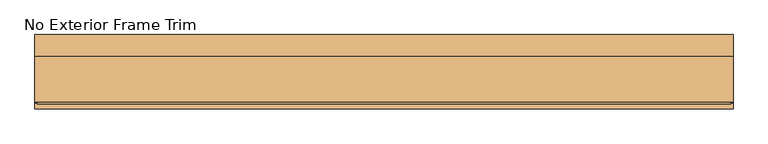
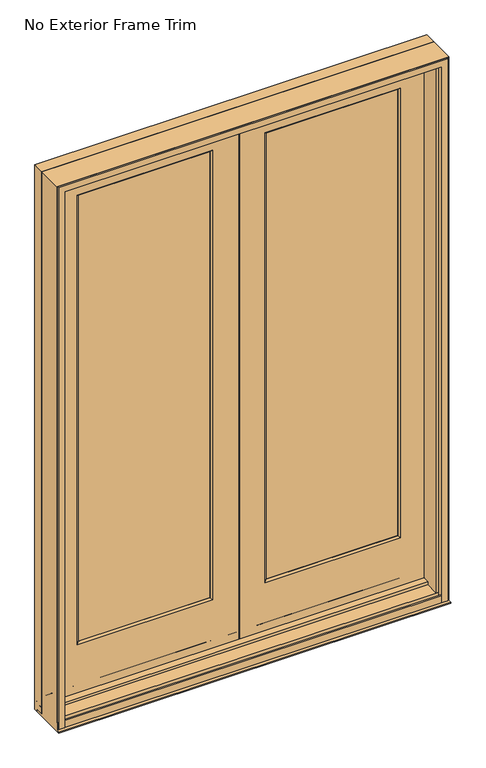
"""IFC4 building model written with IfcOpenShell, lengths in millimetres: door geometry, Door-In_Swing-Milgard-Essence-2_Panel : No Exterior Frame Trim."""

from ifc_helpers import new_model, si_unit, frame, origin, place, context, project, spatial, polyline, outline, extrude, faceted_brep, source, transform, mapped, element, save


def no_exterior_frame_trim_7f6cfa7b(model_context):
    return source(origin(), model_context, "Body", "SolidModel", [
        extrude(outline(polyline([(591.4684989, 28.575), (54.2422052, 28.575), (54.2422052, 53.975), (591.4684989, 53.975), (591.4684989, 28.575)])), frame((0.0, 0.0, 245.0465023), z_axis=(0.0, 0.0, 1.0), x_axis=(1.0, 0.0, 0.0)), (0.0, 0.0, 1.0), 1856.965426),
        faceted_brep([(-22.501829, 56.3244996, 39.0524923), (-39.8139839, 56.3244996, 39.0524923), (-39.8139839, 64.6430002, 39.0524923), (685.524688, 64.6430002, 39.0524923), (685.524688, 56.3244996, 39.0524923), (668.2125331, 56.3244996, 39.0524923), (665.7443122, 53.2765006, 39.0524923), (597.9581931, 53.2765006, 39.0524923), (597.9581931, 55.0418002, 39.0524923), (583.7647037, 55.0418002, 39.0524923), (582.2411552, 53.975, 39.0524923), (578.7581009, 53.975, 39.0524923), (578.7581009, 55.857139, 39.0524923), (579.0279319, 56.3244996, 39.0524923), (66.6827722, 56.3244996, 39.0524923), (66.9526032, 55.857139, 39.0524923), (66.9526032, 53.975, 39.0524923), (63.4695489, 53.975, 39.0524923), (61.9460004, 55.0418002, 39.0524923), (47.7525111, 55.0418002, 39.0524923), (47.7525111, 53.2765006, 39.0524923), (-20.0336081, 53.2765006, 39.0524923), (-22.501829, 56.3244996, 2178.7559624), (-22.501829, 56.3244996, 257.4235308), (-22.1233678, 55.857139, 257.6933617), (-20.5992417, 53.975, 257.6933617), (-20.5992417, 53.975, 254.2103075), (-21.4631194, 55.0418002, 252.686759), (-21.4631194, 55.0418002, 238.4932696), (-20.0336081, 53.2765006, 238.4932696), (-20.0336081, 53.2765006, 2176.2877415), (-20.0336081, 53.2765006, 58.8285873), (-22.501829, 56.3244996, 56.3603664), (47.7525111, 53.2765006, 58.8285873), (597.9581931, 53.2765006, 58.8285873), (665.7443122, 53.2765006, 58.8285873), (685.524688, 53.2765006, 58.8285873), (685.524688, 53.2765006, 238.4932696), (665.7443122, 53.2765006, 238.4932696), (665.7443122, 53.2765006, 2176.2877415), (-39.8139839, 53.2765006, 238.4932696), (-39.8139839, 53.2765006, 58.8285873), (47.7525111, 53.2765006, 2108.5016224), (597.9581931, 53.2765006, 2108.5016224), (597.9581931, 53.2765006, 238.4932696), (47.7525111, 53.2765006, 238.4932696), (47.7525111, 55.0418002, 238.4932696), (47.7525111, 55.0418002, 252.686759), (47.7525111, 53.975, 254.2103075), (47.7525111, 53.975, 257.6933617), (47.7525111, 55.0418002, 257.6933617), (47.7525111, 55.0418002, 2108.5016224), (47.7525111, 55.0418002, 57.3990759), (597.9581931, 55.0418002, 57.3990759), (583.7647037, 55.0418002, 57.3990759), (61.9460004, 55.0418002, 238.4932696), (61.9460004, 55.0418002, 252.686759), (61.9460004, 55.0418002, 257.6933617), (61.9460004, 55.0418002, 2094.3081331), (583.7647037, 55.0418002, 2094.3081331), (583.7647037, 55.0418002, 257.6933617), (597.9581931, 55.0418002, 257.6933617), (597.9581931, 55.0418002, 2108.5016224), (597.9581931, 55.0418002, 252.686759), (583.7647037, 55.0418002, 252.686759), (583.7647037, 55.0418002, 238.4932696), (597.9581931, 55.0418002, 238.4932696), (61.9460004, 55.0418002, 57.3990759), (63.4695489, 53.975, 238.4932696), (63.4695489, 53.975, 254.2103075), (63.4695489, 53.975, 257.6933617), (63.4695489, 53.975, 2092.7845845), (63.4695489, 53.975, 58.2629537), (582.2411552, 53.975, 58.2629537), (578.7581009, 53.975, 58.2629537), (66.9526032, 53.975, 238.4932696), (66.9526032, 53.975, 254.2103075), (578.7581009, 53.975, 254.2103075), (578.7581009, 53.975, 238.4932696), (582.2411552, 53.975, 238.4932696), (582.2411552, 53.975, 254.2103075), (597.9581931, 53.975, 254.2103075), (597.9581931, 53.975, 257.6933617), (582.2411552, 53.975, 257.6933617), (582.2411552, 53.975, 2092.7845845), (66.9526032, 53.975, 2089.3015303), (578.7581009, 53.975, 2089.3015303), (578.7581009, 53.975, 257.6933617), (66.9526032, 53.975, 257.6933617), (685.524688, 53.975, 257.6933617), (666.3099458, 53.975, 257.6933617), (666.3099458, 53.975, 254.2103075), (685.524688, 53.975, 254.2103075), (66.9526032, 53.975, 58.2629537), (-39.8139839, 53.975, 254.2103075), (-39.8139839, 53.975, 257.6933617), (66.9526032, 55.0418002, 238.4932696), (66.9526032, 55.0418002, 252.686759), (66.9526032, 55.857139, 257.6933617), (66.9526032, 55.857139, 2089.3015303), (66.9526032, 55.857139, 56.7388275), (66.6827722, 56.3244996, 56.3603664), (62.3383529, 63.8492502, 253.0791115), (62.3383529, 63.8492502, 2093.9157805), (597.9581931, 63.8492502, 2108.5016224), (597.9581931, 63.8492502, 238.4932696), (47.7525111, 63.8492502, 238.4932696), (47.7525111, 63.8492502, 2108.5016224), (583.3723512, 63.8492502, 253.0791115), (583.3723512, 63.8492502, 2093.9157805), (47.7525111, 64.6430002, 238.4932696), (47.7525111, 64.6430002, 2108.5016224), (-39.8139839, 64.6430002, 2196.0681173), (685.524688, 64.6430002, 2196.0681173), (597.9581931, 64.6430002, 2108.5016224), (597.9581931, 64.6430002, 238.4932696), (-39.8139839, 56.3244996, 56.3603664), (-39.8139839, 55.0418002, 238.4932696), (-39.8139839, 55.0418002, 252.686759), (-39.8139839, 55.857139, 257.6933617), (-39.8139839, 56.3244996, 257.4235308), (-39.8139839, 56.3244996, 2196.0681173), (685.524688, 56.3244996, 56.3603664), (668.2125331, 56.3244996, 56.3603664), (668.2125331, 56.3244996, 2178.7559624), (668.2125331, 56.3244996, 257.4235308), (685.524688, 56.3244996, 257.4235308), (685.524688, 56.3244996, 2196.0681173), (578.7581009, 55.857139, 2089.3015303), (667.1738236, 55.0418002, 238.4932696), (667.1738236, 55.0418002, 252.686759), (667.8340719, 55.857139, 257.6933617), (578.7581009, 55.857139, 56.7388275), (578.7581009, 55.0418002, 252.686759), (578.7581009, 55.0418002, 238.4932696), (578.7581009, 55.857139, 257.6933617), (579.0279319, 56.3244996, 56.3603664), (685.524688, 55.857139, 257.6933617), (685.524688, 55.0418002, 252.686759), (685.524688, 55.0418002, 238.4932696)], [[[0, 1, 2, 3, 4, 5, 6, 7, 8, 9, 10, 11, 12, 13, 14, 15, 16, 17, 18, 19, 20, 21]], [[22, 23, 24, 25, 26, 27, 28, 29, 30]], [[21, 31, 32, 0]], [[20, 33, 34, 7, 6, 35, 36, 37, 38, 39, 30, 29, 40, 41, 31, 21], [42, 43, 44, 45]], [[42, 45, 46, 47, 48, 49, 50, 51]], [[19, 52, 33, 20]], [[8, 53, 54, 9]], [[46, 55, 56, 47]], [[51, 50, 57, 58, 59, 60, 61, 62]], [[63, 64, 65, 66]], [[18, 67, 52, 19]], [[55, 68, 69, 56]], [[58, 57, 70, 71]], [[17, 72, 67, 18]], [[10, 73, 74, 11]], [[71, 70, 49, 48, 69, 68, 75, 76, 77, 78, 79, 80, 81, 82, 83, 84], [85, 86, 87, 88]], [[89, 90, 91, 92]], [[16, 93, 72, 17]], [[94, 26, 25, 95]], [[75, 96, 97, 76]], [[85, 88, 98, 99]], [[15, 100, 93, 16]], [[14, 101, 100, 15]], [[99, 98, 102, 103]], [[104, 105, 106, 107], [103, 102, 108, 109]], [[106, 110, 111, 107]], [[2, 112, 113, 3], [114, 111, 110, 115]], [[1, 116, 41, 40, 117, 118, 94, 95, 119, 120, 121, 112, 2]], [[0, 32, 116, 1]], [[4, 122, 123, 5]], [[121, 120, 23, 22, 124, 125, 126, 127]], [[30, 39, 124, 22]], [[42, 51, 62, 43]], [[58, 71, 84, 59]], [[85, 99, 128, 86]], [[103, 109, 128, 99]], [[107, 111, 114, 104]], [[112, 121, 127, 113]], [[39, 38, 129, 130, 91, 90, 131, 125, 124]], [[5, 123, 35, 6]], [[62, 61, 82, 81, 63, 66, 44, 43]], [[7, 34, 53, 8]], [[84, 83, 60, 59]], [[9, 54, 73, 10]], [[79, 65, 64, 80]], [[11, 74, 132, 12]], [[77, 133, 134, 78]], [[128, 135, 87, 86]], [[109, 108, 135, 128]], [[12, 132, 136, 13]], [[114, 115, 105, 104]], [[127, 126, 137, 89, 92, 138, 139, 37, 36, 122, 4, 3, 113]], [[105, 115, 110, 106]], [[102, 98, 135, 108]], [[126, 125, 131, 137]], [[119, 24, 23, 120]], [[70, 57, 50, 49]], [[95, 25, 24, 119]], [[82, 61, 60, 83]], [[87, 135, 98, 88]], [[137, 131, 90, 89]], [[48, 47, 56, 69]], [[76, 97, 133, 77]], [[80, 64, 63, 81]], [[92, 91, 130, 138]], [[118, 27, 26, 94]], [[97, 96, 134, 133]], [[138, 130, 129, 139]], [[117, 28, 27, 118]], [[40, 29, 28, 117]], [[44, 66, 65, 79, 78, 134, 96, 75, 68, 55, 46, 45]], [[139, 129, 38, 37]], [[33, 52, 67, 72, 93, 100, 101, 136, 132, 74, 73, 54, 53, 34]], [[116, 32, 31, 41]], [[36, 35, 123, 122]], [[13, 136, 101, 14]]]),
        faceted_brep([(-39.8139839, 20.1929984, 39.0524923), (-39.8139839, 20.1929984, 2196.0681173), (-39.8139839, 56.3244996, 2196.0681173), (-39.8139839, 56.3244996, 39.0524923), (685.524688, 56.3244996, 39.0524923), (685.524688, 56.3244996, 2196.0681173), (685.524688, 20.1929984, 2196.0681173), (685.524688, 20.1929984, 39.0524923), (66.7863819, 27.3270033, 257.5271404), (59.6523769, 20.1929984, 250.3931355), (586.0583272, 20.1929984, 250.3931355), (578.9243222, 27.3270033, 257.5271404), (59.6523769, 20.1929984, 2096.6017565), (586.0583272, 20.1929984, 2096.6017565), (669.6356705, 56.3244996, 55.4786786), (669.6356705, 56.3244996, 2180.1790999), (-23.9249664, 56.3244996, 2180.1790999), (-23.9249664, 56.3244996, 55.4786786), (-20.8769674, 53.2765006, 57.9468995), (666.5876715, 53.2765006, 57.9468995), (666.5876715, 53.2765006, 2177.1311009), (-20.8769674, 53.2765006, 2177.1311009), (594.7531877, 53.2765006, 241.698275), (594.7531877, 53.2765006, 2105.296617), (50.9575164, 53.2765006, 2105.296617), (50.9575164, 53.2765006, 241.698275), (50.9575164, 50.8481081, 241.698275), (594.7531877, 50.8481081, 241.698275), (49.0643221, 50.8481081, 2107.1898114), (49.0643221, 50.8481081, 239.8050807), (596.646382, 50.8481081, 239.8050807), (596.646382, 50.8481081, 2107.1898114), (50.9575164, 50.8481081, 2105.296617), (594.7531877, 50.8481081, 2105.296617), (47.7525111, 46.8107689, 238.4932696), (597.9581931, 46.8107689, 238.4932696), (47.7525111, 27.8384005, 238.4932696), (64.012343, 27.8384005, 238.4932696), (64.7489425, 28.575, 238.4932696), (66.7863819, 28.575, 238.4932696), (66.7863819, 27.8384005, 238.4932696), (578.9243222, 27.8384005, 238.4932696), (578.9243222, 28.575, 238.4932696), (580.9617616, 28.575, 238.4932696), (581.6983611, 27.8384005, 238.4932696), (597.9581931, 27.8384005, 238.4932696), (581.6983611, 27.8384005, 254.7531016), (597.9581931, 27.8384005, 254.7531016), (66.7863819, 27.8384005, 254.7531016), (578.9243222, 27.8384005, 254.7531016), (47.7525111, 27.8384005, 254.7531016), (64.012343, 27.8384005, 254.7531016), (47.7525111, 28.575, 255.4897011), (64.7489425, 28.575, 255.4897011), (66.7863819, 28.575, 255.4897011), (578.9243222, 28.575, 255.4897011), (580.9617616, 28.575, 255.4897011), (597.9581931, 28.575, 255.4897011), (47.7525111, 28.575, 257.5271404), (64.7489425, 28.575, 257.5271404), (64.7489425, 28.575, 2091.505191), (580.9617616, 28.575, 2091.505191), (580.9617616, 28.575, 257.5271404), (597.9581931, 28.575, 257.5271404), (578.9243222, 28.575, 257.5271404), (578.9243222, 28.575, 2089.4677516), (66.7863819, 28.575, 2089.4677516), (66.7863819, 28.575, 257.5271404), (581.6983611, 27.8384005, 257.5271404), (597.9581931, 27.8384005, 257.5271404), (47.7525111, 27.8384005, 257.5271404), (64.012343, 27.8384005, 257.5271404), (66.7863819, 27.3270033, 2089.4677516), (64.012343, 27.8384005, 2092.2417904), (47.7525111, 27.8384005, 2108.5016224), (597.9581931, 27.8384005, 2108.5016224), (581.6983611, 27.8384005, 2092.2417904), (47.7525111, 46.8107689, 2108.5016224), (578.9243222, 27.3270033, 2089.4677516), (597.9581931, 46.8107689, 2108.5016224)], [[[0, 1, 2, 3]], [[4, 5, 6, 7]], [[8, 9, 10, 11]], [[0, 7, 6, 1], [9, 12, 13, 10]], [[4, 7, 0, 3]], [[2, 5, 4, 3], [14, 15, 16, 17]], [[17, 18, 19, 14]], [[20, 19, 18, 21], [22, 23, 24, 25]], [[25, 26, 27, 22]], [[28, 29, 30, 31], [26, 32, 33, 27]], [[29, 34, 35, 30]], [[34, 36, 37, 38, 39, 40, 41, 42, 43, 44, 45, 35]], [[44, 46, 47, 45]], [[40, 48, 49, 41]], [[36, 50, 51, 37]], [[50, 52, 53, 51]], [[48, 54, 55, 49]], [[46, 56, 57, 47]], [[52, 58, 59, 60, 61, 62, 63, 57, 56, 43, 42, 55, 54, 39, 38, 53], [64, 65, 66, 67]], [[11, 64, 67, 8]], [[62, 68, 69, 63]], [[58, 70, 71, 59]], [[12, 9, 8, 72]], [[54, 48, 40, 39]], [[72, 8, 67, 66]], [[38, 37, 51, 53]], [[60, 59, 71, 73]], [[73, 71, 70, 74, 75, 69, 68, 76]], [[74, 70, 58, 52, 50, 36, 34, 77]], [[77, 34, 29, 28]], [[32, 26, 25, 24]], [[18, 17, 16, 21]], [[12, 72, 78, 13]], [[66, 65, 78, 72]], [[60, 73, 76, 61]], [[74, 77, 79, 75]], [[28, 31, 79, 77]], [[32, 24, 23, 33]], [[21, 16, 15, 20]], [[6, 5, 2, 1]], [[78, 11, 10, 13]], [[42, 41, 49, 55]], [[65, 64, 11, 78]], [[56, 46, 44, 43]], [[76, 68, 62, 61]], [[79, 35, 45, 47, 57, 63, 69, 75]], [[30, 35, 79, 31]], [[23, 22, 27, 33]], [[15, 14, 19, 20]]]),
        extrude(outline(polyline([(-675.754549, 28.575), (-675.754549, 53.975), (-138.5282552, 53.975), (-138.5282552, 28.575), (-675.754549, 28.575)])), frame((0.0, 0.0, 245.0465023), z_axis=(0.0, 0.0, 1.0), x_axis=(1.0, 0.0, 0.0)), (0.0, 0.0, 1.0), 1856.965426),
        faceted_brep([(-61.784221, 56.3244996, 39.0524923), (-64.252442, 53.2765006, 39.0524923), (-132.0385611, 53.2765006, 39.0524923), (-132.0385611, 55.0418002, 39.0524923), (-146.2320504, 55.0418002, 39.0524923), (-147.755599, 53.975, 39.0524923), (-151.2386532, 53.975, 39.0524923), (-151.2386532, 55.857139, 39.0524923), (-150.9688223, 56.3244996, 39.0524923), (-663.3139819, 56.3244996, 39.0524923), (-663.044151, 55.857139, 39.0524923), (-663.044151, 53.975, 39.0524923), (-666.5272052, 53.975, 39.0524923), (-668.0507537, 55.0418002, 39.0524923), (-682.2442431, 55.0418002, 39.0524923), (-682.2442431, 53.2765006, 39.0524923), (-750.0303622, 53.2765006, 39.0524923), (-752.4985831, 56.3244996, 39.0524923), (-769.810738, 56.3244996, 39.0524923), (-769.810738, 64.6430002, 39.0524923), (-44.4720661, 64.6430002, 39.0524923), (-44.4720661, 56.3244996, 39.0524923), (-61.784221, 56.3244996, 56.3603664), (-64.252442, 53.2765006, 58.8285873), (-61.784221, 56.3244996, 2178.7559624), (-64.252442, 53.2765006, 2176.2877415), (-64.252442, 53.2765006, 238.4932696), (-62.8229306, 55.0418002, 238.4932696), (-62.8229306, 55.0418002, 252.686759), (-63.6868083, 53.975, 254.2103075), (-63.6868083, 53.975, 257.6933617), (-62.1626822, 55.857139, 257.6933617), (-61.784221, 56.3244996, 257.4235308), (-44.4720661, 53.2765006, 58.8285873), (-44.4720661, 53.2765006, 238.4932696), (-750.0303622, 53.2765006, 2176.2877415), (-750.0303622, 53.2765006, 238.4932696), (-769.810738, 53.2765006, 238.4932696), (-769.810738, 53.2765006, 58.8285873), (-750.0303622, 53.2765006, 58.8285873), (-682.2442431, 53.2765006, 58.8285873), (-132.0385611, 53.2765006, 58.8285873), (-132.0385611, 53.2765006, 2108.5016224), (-132.0385611, 53.2765006, 238.4932696), (-682.2442431, 53.2765006, 238.4932696), (-682.2442431, 53.2765006, 2108.5016224), (-132.0385611, 55.0418002, 57.3990759), (-132.0385611, 55.0418002, 2108.5016224), (-132.0385611, 55.0418002, 257.6933617), (-132.0385611, 53.975, 257.6933617), (-132.0385611, 53.975, 254.2103075), (-132.0385611, 55.0418002, 252.686759), (-132.0385611, 55.0418002, 238.4932696), (-668.0507537, 55.0418002, 57.3990759), (-682.2442431, 55.0418002, 57.3990759), (-146.2320504, 55.0418002, 57.3990759), (-682.2442431, 55.0418002, 2108.5016224), (-682.2442431, 55.0418002, 257.6933617), (-668.0507537, 55.0418002, 257.6933617), (-668.0507537, 55.0418002, 2094.3081331), (-146.2320504, 55.0418002, 2094.3081331), (-146.2320504, 55.0418002, 257.6933617), (-146.2320504, 55.0418002, 252.686759), (-146.2320504, 55.0418002, 238.4932696), (-682.2442431, 55.0418002, 252.686759), (-682.2442431, 55.0418002, 238.4932696), (-668.0507537, 55.0418002, 238.4932696), (-668.0507537, 55.0418002, 252.686759), (-147.755599, 53.975, 58.2629537), (-147.755599, 53.975, 2092.7845845), (-147.755599, 53.975, 257.6933617), (-147.755599, 53.975, 254.2103075), (-147.755599, 53.975, 238.4932696), (-663.044151, 53.975, 58.2629537), (-666.5272052, 53.975, 58.2629537), (-151.2386532, 53.975, 58.2629537), (-666.5272052, 53.975, 2092.7845845), (-666.5272052, 53.975, 257.6933617), (-682.2442431, 53.975, 257.6933617), (-682.2442431, 53.975, 254.2103075), (-666.5272052, 53.975, 254.2103075), (-666.5272052, 53.975, 238.4932696), (-663.044151, 53.975, 238.4932696), (-663.044151, 53.975, 254.2103075), (-151.2386532, 53.975, 254.2103075), (-151.2386532, 53.975, 238.4932696), (-151.2386532, 53.975, 2089.3015303), (-151.2386532, 53.975, 257.6933617), (-663.044151, 53.975, 257.6933617), (-663.044151, 53.975, 2089.3015303), (-44.4720661, 53.975, 254.2103075), (-44.4720661, 53.975, 257.6933617), (-769.810738, 53.975, 257.6933617), (-769.810738, 53.975, 254.2103075), (-750.5959958, 53.975, 254.2103075), (-750.5959958, 53.975, 257.6933617), (-151.2386532, 55.857139, 56.7388275), (-151.2386532, 55.857139, 2089.3015303), (-151.2386532, 55.857139, 257.6933617), (-151.2386532, 55.0418002, 252.686759), (-151.2386532, 55.0418002, 238.4932696), (-150.9688223, 56.3244996, 56.3603664), (-146.624403, 63.8492502, 2093.9157805), (-146.624403, 63.8492502, 253.0791115), (-682.2442431, 63.8492502, 2108.5016224), (-132.0385611, 63.8492502, 2108.5016224), (-132.0385611, 63.8492502, 238.4932696), (-682.2442431, 63.8492502, 238.4932696), (-667.6584012, 63.8492502, 2093.9157805), (-667.6584012, 63.8492502, 253.0791115), (-132.0385611, 64.6430002, 2108.5016224), (-132.0385611, 64.6430002, 238.4932696), (-769.810738, 64.6430002, 2196.0681173), (-44.4720661, 64.6430002, 2196.0681173), (-682.2442431, 64.6430002, 2108.5016224), (-682.2442431, 64.6430002, 238.4932696), (-44.4720661, 56.3244996, 2196.0681173), (-44.4720661, 56.3244996, 257.4235308), (-44.4720661, 55.857139, 257.6933617), (-44.4720661, 55.0418002, 252.686759), (-44.4720661, 55.0418002, 238.4932696), (-44.4720661, 56.3244996, 56.3603664), (-752.4985831, 56.3244996, 56.3603664), (-769.810738, 56.3244996, 56.3603664), (-769.810738, 56.3244996, 2196.0681173), (-769.810738, 56.3244996, 257.4235308), (-752.4985831, 56.3244996, 257.4235308), (-752.4985831, 56.3244996, 2178.7559624), (-663.044151, 55.857139, 2089.3015303), (-752.120122, 55.857139, 257.6933617), (-751.4598736, 55.0418002, 252.686759), (-751.4598736, 55.0418002, 238.4932696), (-663.044151, 55.857139, 56.7388275), (-663.044151, 55.857139, 257.6933617), (-663.044151, 55.0418002, 238.4932696), (-663.044151, 55.0418002, 252.686759), (-663.3139819, 56.3244996, 56.3603664), (-769.810738, 55.0418002, 238.4932696), (-769.810738, 55.0418002, 252.686759), (-769.810738, 55.857139, 257.6933617)], [[[0, 1, 2, 3, 4, 5, 6, 7, 8, 9, 10, 11, 12, 13, 14, 15, 16, 17, 18, 19, 20, 21]], [[1, 0, 22, 23]], [[24, 25, 26, 27, 28, 29, 30, 31, 32]], [[2, 1, 23, 33, 34, 26, 25, 35, 36, 37, 38, 39, 16, 15, 40, 41], [42, 43, 44, 45]], [[3, 2, 41, 46]], [[42, 47, 48, 49, 50, 51, 52, 43]], [[14, 13, 53, 54]], [[4, 3, 46, 55]], [[47, 56, 57, 58, 59, 60, 61, 48]], [[52, 51, 62, 63]], [[64, 65, 66, 67]], [[5, 4, 55, 68]], [[60, 69, 70, 61]], [[63, 62, 71, 72]], [[12, 11, 73, 74]], [[6, 5, 68, 75]], [[69, 76, 77, 78, 79, 80, 81, 82, 83, 84, 85, 72, 71, 50, 49, 70], [86, 87, 88, 89]], [[90, 91, 30, 29]], [[92, 93, 94, 95]], [[7, 6, 75, 96]], [[86, 97, 98, 87]], [[85, 84, 99, 100]], [[8, 7, 96, 101]], [[97, 102, 103, 98]], [[104, 105, 106, 107], [102, 108, 109, 103]], [[106, 105, 110, 111]], [[20, 19, 112, 113], [114, 115, 111, 110]], [[21, 20, 113, 116, 117, 118, 91, 90, 119, 120, 34, 33, 121]], [[0, 21, 121, 22]], [[18, 17, 122, 123]], [[116, 124, 125, 126, 127, 24, 32, 117]], [[25, 24, 127, 35]], [[42, 45, 56, 47]], [[60, 59, 76, 69]], [[86, 89, 128, 97]], [[102, 97, 128, 108]], [[105, 104, 114, 110]], [[113, 112, 124, 116]], [[17, 16, 39, 122]], [[35, 127, 126, 129, 95, 94, 130, 131, 36]], [[15, 14, 54, 40]], [[56, 45, 44, 65, 64, 79, 78, 57]], [[13, 12, 74, 53]], [[81, 80, 67, 66]], [[76, 59, 58, 77]], [[11, 10, 132, 73]], [[128, 89, 88, 133]], [[83, 82, 134, 135]], [[10, 9, 136, 132]], [[108, 128, 133, 109]], [[114, 104, 107, 115]], [[124, 112, 19, 18, 123, 38, 37, 137, 138, 93, 92, 139, 125]], [[107, 106, 111, 115]], [[118, 117, 32, 31]], [[125, 139, 129, 126]], [[103, 109, 133, 98]], [[70, 49, 48, 61]], [[78, 77, 58, 57]], [[88, 87, 98, 133]], [[91, 118, 31, 30]], [[139, 92, 95, 129]], [[119, 90, 29, 28]], [[93, 138, 130, 94]], [[50, 71, 62, 51]], [[84, 83, 135, 99]], [[80, 79, 64, 67]], [[120, 119, 28, 27]], [[138, 137, 131, 130]], [[99, 135, 134, 100]], [[44, 43, 52, 63, 72, 85, 100, 134, 82, 81, 66, 65]], [[34, 120, 27, 26]], [[137, 37, 36, 131]], [[121, 33, 23, 22]], [[38, 123, 122, 39]], [[41, 40, 54, 53, 74, 73, 132, 136, 101, 96, 75, 68, 55, 46]], [[9, 8, 101, 136]]]),
        faceted_brep([(-44.4720661, 20.1929984, 39.0524923), (-44.4720661, 56.3244996, 39.0524923), (-44.4720661, 56.3244996, 2196.0681173), (-44.4720661, 20.1929984, 2196.0681173), (-769.810738, 56.3244996, 39.0524923), (-769.810738, 20.1929984, 39.0524923), (-769.810738, 20.1929984, 2196.0681173), (-769.810738, 56.3244996, 2196.0681173), (-151.0724319, 27.3270033, 257.5271404), (-663.2103723, 27.3270033, 257.5271404), (-670.3443772, 20.1929984, 250.3931355), (-143.938427, 20.1929984, 250.3931355), (-670.3443772, 20.1929984, 2096.6017565), (-143.938427, 20.1929984, 2096.6017565), (-753.9217206, 56.3244996, 55.4786786), (-60.3610836, 56.3244996, 55.4786786), (-60.3610836, 56.3244996, 2180.1790999), (-753.9217206, 56.3244996, 2180.1790999), (-750.8737216, 53.2765006, 57.9468995), (-63.4090826, 53.2765006, 57.9468995), (-750.8737216, 53.2765006, 2177.1311009), (-63.4090826, 53.2765006, 2177.1311009), (-679.0392377, 53.2765006, 241.698275), (-135.2435664, 53.2765006, 241.698275), (-135.2435664, 53.2765006, 2105.296617), (-679.0392377, 53.2765006, 2105.296617), (-679.0392377, 50.8481081, 241.698275), (-135.2435664, 50.8481081, 241.698275), (-133.3503721, 50.8481081, 2107.1898114), (-680.9324321, 50.8481081, 2107.1898114), (-680.9324321, 50.8481081, 239.8050807), (-133.3503721, 50.8481081, 239.8050807), (-679.0392377, 50.8481081, 2105.296617), (-135.2435664, 50.8481081, 2105.296617), (-682.2442431, 46.8107689, 238.4932696), (-132.0385611, 46.8107689, 238.4932696), (-682.2442431, 27.8384005, 238.4932696), (-665.9844111, 27.8384005, 238.4932696), (-665.2478116, 28.575, 238.4932696), (-663.2103723, 28.575, 238.4932696), (-663.2103723, 27.8384005, 238.4932696), (-151.0724319, 27.8384005, 238.4932696), (-151.0724319, 28.575, 238.4932696), (-149.0349925, 28.575, 238.4932696), (-148.298393, 27.8384005, 238.4932696), (-132.0385611, 27.8384005, 238.4932696), (-148.298393, 27.8384005, 254.7531016), (-132.0385611, 27.8384005, 254.7531016), (-663.2103723, 27.8384005, 254.7531016), (-151.0724319, 27.8384005, 254.7531016), (-682.2442431, 27.8384005, 254.7531016), (-665.9844111, 27.8384005, 254.7531016), (-149.0349925, 28.575, 255.4897011), (-132.0385611, 28.575, 255.4897011), (-663.2103723, 28.575, 255.4897011), (-151.0724319, 28.575, 255.4897011), (-682.2442431, 28.575, 255.4897011), (-665.2478116, 28.575, 255.4897011), (-682.2442431, 28.575, 257.5271404), (-665.2478116, 28.575, 257.5271404), (-665.2478116, 28.575, 2091.505191), (-149.0349925, 28.575, 2091.505191), (-149.0349925, 28.575, 257.5271404), (-132.0385611, 28.575, 257.5271404), (-663.2103723, 28.575, 257.5271404), (-151.0724319, 28.575, 257.5271404), (-151.0724319, 28.575, 2089.4677516), (-663.2103723, 28.575, 2089.4677516), (-148.298393, 27.8384005, 257.5271404), (-132.0385611, 27.8384005, 257.5271404), (-682.2442431, 27.8384005, 257.5271404), (-665.9844111, 27.8384005, 257.5271404), (-151.0724319, 27.3270033, 2089.4677516), (-148.298393, 27.8384005, 2092.2417904), (-665.9844111, 27.8384005, 2092.2417904), (-682.2442431, 27.8384005, 2108.5016224), (-132.0385611, 27.8384005, 2108.5016224), (-132.0385611, 46.8107689, 2108.5016224), (-663.2103723, 27.3270033, 2089.4677516), (-682.2442431, 46.8107689, 2108.5016224)], [[[0, 1, 2, 3]], [[4, 5, 6, 7]], [[8, 9, 10, 11]], [[0, 3, 6, 5], [11, 10, 12, 13]], [[4, 1, 0, 5]], [[2, 1, 4, 7], [14, 15, 16, 17]], [[15, 14, 18, 19]], [[20, 21, 19, 18], [22, 23, 24, 25]], [[23, 22, 26, 27]], [[28, 29, 30, 31], [27, 26, 32, 33]], [[31, 30, 34, 35]], [[35, 34, 36, 37, 38, 39, 40, 41, 42, 43, 44, 45]], [[45, 44, 46, 47]], [[41, 40, 48, 49]], [[37, 36, 50, 51]], [[47, 46, 52, 53]], [[49, 48, 54, 55]], [[51, 50, 56, 57]], [[53, 52, 43, 42, 55, 54, 39, 38, 57, 56, 58, 59, 60, 61, 62, 63], [64, 65, 66, 67]], [[9, 8, 65, 64]], [[63, 62, 68, 69]], [[59, 58, 70, 71]], [[13, 72, 8, 11]], [[55, 42, 41, 49]], [[72, 66, 65, 8]], [[43, 52, 46, 44]], [[61, 73, 68, 62]], [[73, 74, 71, 70, 75, 76, 69, 68]], [[76, 77, 35, 45, 47, 53, 63, 69]], [[77, 28, 31, 35]], [[33, 24, 23, 27]], [[19, 21, 16, 15]], [[13, 12, 78, 72]], [[66, 72, 78, 67]], [[61, 60, 74, 73]], [[76, 75, 79, 77]], [[28, 77, 79, 29]], [[33, 32, 25, 24]], [[21, 20, 17, 16]], [[6, 3, 2, 7]], [[78, 12, 10, 9]], [[39, 54, 48, 40]], [[67, 78, 9, 64]], [[74, 60, 59, 71]], [[57, 38, 37, 51]], [[79, 75, 70, 58, 56, 50, 36, 34]], [[30, 29, 79, 34]], [[25, 32, 26, 22]], [[17, 20, 18, 14]]]),
        faceted_brep([(719.8791802, 74.6125, 0.0), (719.8791802, 74.6125, 2235.2), (719.8791802, 27.6987011, 2235.2), (719.8791802, 27.7018482, 9.128125), (719.8791802, 61.9125011, 9.128125), (719.8791802, 61.9125011, 0.0), (-804.1208198, 61.9125011, 0.0), (-804.1208198, 61.9125011, 9.128125), (-804.1208198, 27.7018482, 9.128125), (-804.1208198, 27.6987011, 2235.2), (-804.1208198, 74.6125, 2235.2), (-804.1208198, 74.6125, 0.0), (-775.5465905, 74.6125, 41.6602461), (691.3049508, 74.6125, 41.6602461), (691.3049508, 74.6125, 2206.6257706), (-775.5465905, 74.6125, 2206.6257706), (688.7641767, 61.9125011, 9.128125), (688.7641767, 61.9125011, 40.5405728), (-773.0058163, 61.9125011, 40.5405728), (-773.0058163, 61.9125011, 9.128125), (693.7179256, 27.7018482, 9.128125), (693.7179256, 50.2285006, 9.128125), (691.304169, 50.2285006, 9.128125), (691.304169, 55.02769, 9.128125), (688.7641767, 55.02769, 9.128125), (-777.9595653, 27.7018482, 9.128125), (-773.0058163, 55.02769, 9.128125), (-775.5458087, 55.02769, 9.128125), (-775.5458087, 50.2285006, 9.128125), (-777.9595653, 50.2285006, 9.128125), (688.7641767, 66.2127992, 41.2988289), (691.3049508, 66.2127992, 41.2988289), (691.3049508, 68.2625043, 41.6602461), (-775.5465905, 68.2625043, 41.6602461), (-775.5465905, 66.2127992, 41.2988289), (-773.0058163, 66.2127992, 41.2988289), (691.3049508, 66.2127992, 2206.6257706), (688.7641767, 66.2127992, 2204.0849965), (-773.0058163, 66.2127992, 2204.0849965), (-775.5465905, 66.2127992, 2206.6257706), (688.7641767, 55.02769, 2204.0849965), (-773.0058163, 55.02769, 2204.0849965), (691.304169, 55.02769, 2206.6249888), (-775.5458087, 55.02769, 2206.6249888), (-777.9595653, 27.6987011, 2209.0380233), (-777.9595653, 50.2285006, 2209.0380233), (693.7179256, 50.2285006, 2209.0380233), (693.7179256, 27.6987011, 2209.0380233), (691.304169, 50.2285006, 2206.6249888), (-775.5458087, 50.2285006, 2206.6249888)], [[[0, 1, 2, 3, 4, 5]], [[6, 7, 8, 9, 10, 11]], [[10, 1, 0, 11], [12, 13, 14, 15]], [[5, 4, 16, 17, 18, 19, 7, 6]], [[5, 6, 11, 0]], [[20, 21, 22, 23, 24, 16, 4, 3]], [[25, 8, 7, 19, 26, 27, 28, 29]], [[17, 30, 31, 32, 33, 34, 35, 18]], [[12, 33, 32, 13]], [[36, 31, 30, 37, 38, 35, 34, 39]], [[37, 40, 41, 38]], [[40, 24, 23, 42, 43, 27, 26, 41]], [[44, 45, 46, 47]], [[2, 9, 8, 25, 44, 47, 20, 3]], [[1, 10, 9, 2]], [[39, 15, 14, 36]], [[13, 32, 31, 36, 14]], [[40, 37, 30, 17, 16, 24]], [[22, 48, 42, 23]], [[21, 46, 45, 29, 28, 49, 48, 22]], [[20, 47, 46, 21]], [[48, 49, 43, 42]], [[15, 39, 34, 33, 12]], [[26, 19, 18, 35, 38, 41]], [[43, 49, 28, 27]], [[29, 45, 44, 25]]]),
        faceted_brep([(719.8791802, -87.2170398, 0.0007738), (719.8791802, 61.9125011, 0.0007738), (719.8791802, 61.9125011, 40.9473783), (719.8791802, 55.5625016, 39.2302591), (719.8791802, 55.5625016, 36.0475021), (719.8791802, 27.7018482, 34.0993068), (719.8791802, 27.7018482, 2235.2), (719.8791802, -72.3899958, 2235.2), (719.8791802, -72.3899958, 33.0268847), (719.8791802, -74.5870975, 32.7181022), (719.8791802, -74.5870975, 4.9752253), (719.8791802, -87.2170398, 3.8703788), (-804.1208198, 61.9125011, 0.0007738), (-804.1208198, -87.2170398, 0.0007738), (-804.1208198, -87.2170398, 3.8703788), (-804.1208198, -74.5870975, 4.9752253), (-804.1208198, -74.5870975, 32.7181022), (-804.1208198, -72.3899958, 33.0268847), (-804.1208198, -72.3899958, 2235.2), (-804.1208198, 27.7018482, 2235.2), (-804.1208198, 27.7018482, 34.0993068), (-804.1208198, 55.5625016, 36.0475021), (-804.1208198, 55.5625016, 39.2302591), (-804.1208198, 61.9125011, 40.9473783), (715.0539447, -74.5870975, 4.9752253), (715.0539447, -76.1999992, 4.8341313), (691.3049508, -76.1999992, 4.8341313), (691.3049508, -74.5870975, 4.9752253), (-775.5465905, -74.5870975, 4.9752253), (-775.5465905, -76.1999992, 4.8341313), (-799.2955843, -76.1999992, 4.8341313), (-799.2955843, -74.5870975, 4.9752253), (-799.2955843, -74.5870975, 32.7181022), (715.0539447, -74.5870975, 32.7181022), (691.3049508, -74.5870975, 32.7181022), (-775.5465905, -74.5870975, 32.7181022), (-799.2955843, -68.8467009, 33.5248623), (-801.9625942, -68.8467009, 33.5248623), (-801.9625942, -72.3899958, 33.0268847), (691.3049508, -68.8467009, 33.5248623), (-775.5465905, -68.8467009, 33.5248623), (717.7209545, -72.3899958, 33.0268847), (717.7209545, -68.8467009, 33.5248623), (715.0539447, -68.8467009, 33.5248623), (691.3049508, -68.8467009, 17.4625), (-775.5465905, -68.8467009, 17.4625), (717.7209545, -68.8467009, 17.4625), (715.0539447, -68.8467009, 17.4625), (-799.2955843, -68.8467009, 17.4625), (-801.9625942, -68.8467009, 17.4625), (691.3049508, -53.8860989, 17.4625), (-775.5465905, -53.8860989, 17.4625), (717.7209545, -65.2779957, 17.4625), (715.0539447, -65.2779957, 17.4625), (-799.2955843, -65.2779957, 17.4625), (-801.9625942, -65.2779957, 17.4625), (691.3049508, -53.8860989, 34.8617092), (-775.5465905, -53.8860989, 34.8617092), (691.3049508, -53.3399975, 34.9482004), (680.1863101, -53.3399975, 34.9482004), (676.9703302, -7.3532983, 42.2315423), (-761.2119699, -7.3532983, 42.2315423), (-764.4279497, -53.3399975, 34.9482004), (-775.5465905, -53.3399975, 34.9482004), (676.9703302, -7.3532983, 53.8407291), (-761.2119699, -7.3532983, 53.8407291), (675.4160732, 14.8717015, 57.7596273), (-759.6577128, 14.8717015, 57.7596273), (678.8330892, 14.8717015, 57.7596273), (678.8330892, 7.5583358, 56.4700734), (681.6271165, 7.5583358, 56.4700734), (681.6271165, 14.8717015, 57.7596273), (-765.8687562, 14.8717015, 57.7596273), (-765.8687562, 7.5583358, 56.4700734), (-763.0747288, 7.5583358, 56.4700734), (-763.0747288, 14.8717015, 57.7596273), (681.6271165, 14.8717015, 33.2021408), (678.8330892, 14.8717015, 33.2021408), (-763.0747288, 14.8717015, 33.2021408), (-765.8687562, 14.8717015, 33.2021408), (675.4160732, 14.8717015, 33.2021408), (-759.6577128, 14.8717015, 33.2021408), (-777.9595653, 27.7018482, 34.0993068), (-777.9595653, 50.295149, 35.6791751), (-775.5465905, 50.295149, 35.6791751), (-775.5465905, 15.6806239, 33.2587058), (-765.8687562, 15.6806239, 33.2587058), (-763.0747288, 15.6806239, 33.2587058), (-759.6011426, 15.6806239, 33.2587058), (675.3595029, 15.6806239, 33.2587058), (678.8330892, 15.6806239, 33.2587058), (681.6271165, 15.6806239, 33.2587058), (691.3049508, 15.6806239, 33.2587058), (691.3049508, 50.295149, 35.6791751), (693.7179256, 50.295149, 35.6791751), (693.7179256, 27.7018482, 34.0993068), (691.3049508, -53.3399975, 2206.6257706), (691.3049508, -76.1999992, 2206.6257706), (715.0539447, -76.1999992, 2230.3747645), (-799.2955843, -76.1999992, 2230.3747645), (-775.5465905, -76.1999992, 2206.6257706), (715.0539447, -65.2779957, 2230.3747645), (717.7209545, -65.2779957, 2233.0417743), (-801.9625942, -65.2779957, 2233.0417743), (-799.2955843, -65.2779957, 2230.3747645), (717.7209545, -72.3899958, 2233.0417743), (-801.9625942, -72.3899958, 2233.0417743), (693.7179256, 27.7018482, 2209.0387455), (-777.9595653, 27.7018482, 2209.0387455), (693.7179256, 50.295149, 2209.0387455), (691.3049508, 50.295149, 2206.6257706), (-775.5465905, 50.295149, 2206.6257706), (-777.9595653, 50.295149, 2209.0387455), (691.3049508, 15.6806239, 2206.6257706), (681.6271165, 15.6806239, 2196.9479363), (-765.8687562, 15.6806239, 2196.9479363), (-775.5465905, 15.6806239, 2206.6257706), (681.6271165, 7.5583358, 2196.9479363), (678.8330892, 7.5583358, 2194.153909), (-763.0747288, 7.5583358, 2194.153909), (-765.8687562, 7.5583358, 2196.9479363), (678.8330892, 15.6806239, 2194.153909), (675.3595029, 15.6806239, 2190.6803228), (-759.6011426, 15.6806239, 2190.6803228), (-763.0747288, 15.6806239, 2194.153909), (680.1863101, -53.3399975, 2195.5071299), (-775.5465905, -53.3399975, 2206.6257706), (-764.4279497, -53.3399975, 2195.5071299)], [[[0, 1, 2, 3, 4, 5, 6, 7, 8, 9, 10, 11]], [[12, 13, 14, 15, 16, 17, 18, 19, 20, 21, 22, 23]], [[11, 14, 13, 0]], [[10, 24, 25, 26, 27, 28, 29, 30, 31, 15, 14, 11]], [[15, 31, 32, 16]], [[9, 33, 24, 10]], [[27, 34, 35, 28]], [[16, 32, 36, 37, 38, 17]], [[34, 39, 40, 35]], [[8, 41, 42, 43, 33, 9]], [[39, 44, 45, 40]], [[42, 46, 47, 43]], [[36, 48, 49, 37]], [[44, 50, 51, 45]], [[46, 52, 53, 47]], [[48, 54, 55, 49]], [[50, 56, 57, 51]], [[56, 58, 59, 60, 61, 62, 63, 57]], [[60, 64, 65, 61]], [[64, 66, 67, 65]], [[68, 69, 70, 71]], [[72, 73, 74, 75]], [[71, 76, 77, 68]], [[75, 78, 79, 72]], [[66, 80, 81, 67]], [[21, 20, 82, 83, 84, 85, 86, 79, 78, 87, 88, 81, 80, 89, 90, 77, 76, 91, 92, 93, 94, 95, 5, 4]], [[3, 22, 21, 4]], [[2, 23, 22, 3]], [[1, 12, 23, 2]], [[12, 1, 0, 13]], [[96, 58, 56, 50, 44, 39, 34, 27, 26, 97]], [[97, 26, 25, 98, 99, 30, 29, 100]], [[98, 25, 24, 33, 43, 47, 53, 101]], [[101, 53, 52, 102, 103, 55, 54, 104]], [[102, 52, 46, 42, 41, 105]], [[105, 41, 8, 7, 18, 17, 38, 106]], [[6, 5, 95, 107, 108, 82, 20, 19]], [[107, 95, 94, 109]], [[109, 94, 93, 110, 111, 84, 83, 112]], [[110, 93, 92, 113]], [[113, 92, 91, 114, 115, 86, 85, 116]], [[114, 91, 76, 71, 70, 117]], [[117, 70, 69, 118, 119, 74, 73, 120]], [[118, 69, 68, 77, 90, 121]], [[121, 90, 89, 122, 123, 88, 87, 124]], [[122, 89, 80, 66, 64, 60, 59, 125]], [[125, 59, 58, 96, 126, 63, 62, 127]], [[97, 100, 126, 96]], [[98, 101, 104, 99]], [[102, 105, 106, 103]], [[7, 6, 19, 18]], [[107, 109, 112, 108]], [[110, 113, 116, 111]], [[114, 117, 120, 115]], [[118, 121, 124, 119]], [[122, 125, 127, 123]], [[100, 29, 28, 35, 40, 45, 51, 57, 63, 126]], [[104, 54, 48, 36, 32, 31, 30, 99]], [[106, 38, 37, 49, 55, 103]], [[112, 83, 82, 108]], [[116, 85, 84, 111]], [[120, 73, 72, 79, 86, 115]], [[124, 87, 78, 75, 74, 119]], [[127, 62, 61, 65, 67, 81, 88, 123]]]),
    ])


if __name__ == "__main__":
    model = new_model("IFC4")
    model_context = context("Model", 3, world=origin())
    ifc_project = project(units=[si_unit("LENGTHUNIT", "METRE", prefix="MILLI")], contexts=[model_context])
    site = spatial("IfcSite", under=ifc_project)
    building = spatial("IfcBuilding", under=site)
    placement = place(None, origin())
    no_exterior_frame_trim_shape = no_exterior_frame_trim_7f6cfa7b(model_context)
    element("IfcDoor", 1, ObjectType="Door-In_Swing-Milgard-Essence-2_Panel : No Exterior Frame Trim", at=placement, inside=building, context=model_context, shape_type="MappedRepresentation", body=[
        mapped(no_exterior_frame_trim_shape, transform((0.0, 0.0, 0.0), x_axis=(1.0, 0.0, 0.0), y_axis=(0.0, 1.0, 0.0), z_axis=(0.0, 0.0, 1.0))),
    ])
    save(model, "model.ifc")

# Revit data of these elements
# Type "Door-In_Swing-Milgard-Essence-2_Panel : No Exterior Frame Trim"
#   Type Mark = "25"
#   Version = "2014 - v1.0a"
#   STC Ratings = ""
#   Product data url = "https://bimobject.com/milgardwindowsanddoors/product/milgard-310"
#   Performance Ratings = "https://www.milgard.com/sites/default/files/new-series/essence-series/essence-series-french-style-sliding-doors/field_series_detail_ratings_file/efsd_performance_chart.pdf"
#   Max/Min Note [instance default] = "MIN (5' x 6' 8'') / MAX (6' x 8')"
#   Installation Service and URL = "https://www.milgard.com/professionals/installation-finishing"
#   Frame Type = "4 9/16'' Wall Condition"
#   Exterior Trim = "Not Available"
#   Copyright = "Copyright © 2017 Milgard Manufacturing Inc. All Rights Reserved."
#   Warranty URL = "https://www.milgard.com/learn/understanding-your-full-lifetime-warranty"
#   Video Link = "https://www.youtube.com/user/MilgardWindows"
#   URL = "https://www.milgard.com"
#   Product Documentation Link = "https://www.milgard.com/professionals/essence-series-patio-doors/essence-series-swing-french-doors-new#series-styles--wrapper"
#   Performance URL = "https://www.milgard.com/sites/default/files/series-detail/files/ratings/essence_is-os_performance_ratings_0.pdf"
#   Material = ""
#   Size Note = "Essence Series doors are custom built to size and specifications"
#   Manufacturer Phone Number = "1-800-Milgard"
#   Manufacturer Address = "1010 54th Avenue East, Tacoma, WA 98424"
#   Keynote = "08 14 00"
#   Product Page URL = "https://www.milgard.com/professionals/essence-series-patio-doors/essence-series-swing-french-doors-new#series-styles--wrapper"
#   Product Name = "Essence Series In-Swing French Door, 2 Panel"
#   Operation = "In-Swing"
#   Model = "Essence"
#   Manufacturer = "Milgard Window & Doors"
#   Inset Note [instance default] = "To set Door into wall use Inset parameter found in Instance Properties."
#   Grid Style [instance default] = "Select ‘Grid Style’"
#   Grid Pattern [instance default] = "Select ‘Grid Pattern'"
#   Description = "In-Swing Door, 2 Panel"
#   Construction Type = "-"
#   Assembly Code = "B2030"
#   Analytic Construction = "<None>"
#   Vent Opening Width [instance default] = 2' - 0.05664"
#   Vent Opening Height [instance default] = 7' - 0"
#   Vent Opening Area - Overall [instance default] = 28.0661 SF
#   Vent Opening Area - Individual [instance default] = 14.033 SF
#   Frame Width [instance default] = 5' - 0"
#   Frame Height [instance default] = 7' - 4"
#   Door Swing [instance default] = 90.00°
#   Daylight Opening Width [instance default] = 1' - 8 3/16"
#   Daylight Opening Height [instance default] = 5' - 11 7/8"
#   Daylight Opening Area - Overall [instance default] = 20.1525 SF
#   Daylight Opening Area - Individual [instance default] = 10.0762 SF
#   Width C Min [instance default] = 5' - 0"
#   Wall Width [instance default] = 1' - 0"
#   Individual Door Panel Width [instance default] = 2' - 4.55664"
#   Individual Door Panel Height [instance default] = 7' - 0 59/64"
#   Jamb Extension [instance default] = 0' - 6 1/16"
#   Height C Min [instance default] = 7' - 4"
#   Thermal Resistance (R) = 1.7611 (m²·K)/W
#   Side to Glazing = 0' - 5 5/128"
#   Rough Width [instance default] = 5' - 1"
#   Rough Offset = 0' - 0 1/2"
#   Rough Height [instance default] = 7' - 4 1/2"
#   Inset Offset [instance default] = 0' - 0"
#   Inset [instance default] = 0' - 0"
#   Height [instance default] = 7' - 4"
#   Heat Transfer Coefficient (U) = 0.567826 W/(m²·K)
#   Glazing Thickness = 0' - 1"
#   Glass Width [instance default] = 1' - 9.11914"
#   Glass Height [instance default] = 6' - 0 13/16"
#   Top to Glazing = 0' - 5 1/8"
#   Width [instance default] = 6' - 0"
#   Call Out Width [instance default] = 5' - 0"
#   Call Out Height [instance default] = 7' - 4"
#   Center to Interior = 0' - 1 5/16"
#   Center to Exterior = 0' - 4 5/8"
#   C Panel Height [instance default] = 7' - 0 59/64"
#   C Panel Width [instance default] = 2' - 4.55664"
#   C Door Swing [instance default] = 90.00°
#   C Brick Mold = 0' - 0"
#   Bottom to Glazing = 0' - 10 1/256"
#   Warning Text [instance default] = yes
#   Overall Min Max [instance default] = no
#   Operation Symbol [instance default] = yes
#   Min Max Text [instance default] = no
#   Grid Visibility C [instance default] = no
#   Ext Flat = no
#   Ext Brickmould = no
#   Jamb Extension by Others [instance default] = no
#   Interior Trim by Others [instance default] = no
#   Grid Style - Simulated Divide Lite (3/4in) [instance default] = no
#   Grid Style - Simulated Divide Lite (2-1/4in) [instance default] = no
#   Grid Style - Simulated Divide Lite (1-1/8in) [instance default] = no
#   Grid Style - Grids Between Glass (5/8in) [instance default] = no
#   Grid Style - Grids Between Glass (1-1/16in) [instance default] = no
#   Grid Pattern - Standard [instance default] = no
#   Flat Trim = no
#   Ext Trim Visible = no
#   Constraint = 1
#   C Jamb Extension Visibility [instance default] = no
#   Brick Mold = no
#   Interior Frame = Wood - Milgard - Douglas Fir
#   Glazing Material = Glass - Milgard - SunCoat Low-E2
#   Exterior Frame = Fiberglass - Milgard - Powder Coat, Frost
#   Visual Light Transmittance = 0
#   Solar Heat Gain Coefficient = 0
#   Wall Closure = (empty or 0)
# Element 1 (IfcDoor, "Door-In_Swing-Milgard-Essence-2_Panel : No Exterior Frame Trim")
#   Wall Width = 0' - 6"
#   Jamb Extension = 0' - 0 1/16"
#   Materials on its faces: "Fiberglass - Milgard - Powder Coat, Frost", "Wood - Milgard - Douglas Fir", "Glass - Milgard - SunCoat Low-E2"
# Materials
#   "Wood - Milgard - Douglas Fir": class "Wood", colour RGB 204 153 0, transparency 0, Keynote = "06 01 00", Model = "Douglas Fir", Manufacturer = "Milgard", URL = "https://www.milgard.com", Description = "Clear Vertical Grain Douglas Fir", Cost = 0
#   "Glass - Milgard - SunCoat Low-E2": class "Glass", colour RGB 218 227 224, transparency 0.7, Keynote = "08 81 00.A1", Model = "Suncoat", Manufacturer = "Milgard", URL = "https://www.milgard.com", Description = "SunCoat Low-E2 Glass", Cost = 0
#   "Fiberglass - Milgard - Powder Coat, Frost": class "Fiberglass", colour RGB 236 242 252, transparency 0, Keynote = "09 91 00.A1", Model = "Frost", Manufacturer = "Milgard", URL = "https://www.milgard.com", Description = "Powder Coat, Frost", Cost = 0
